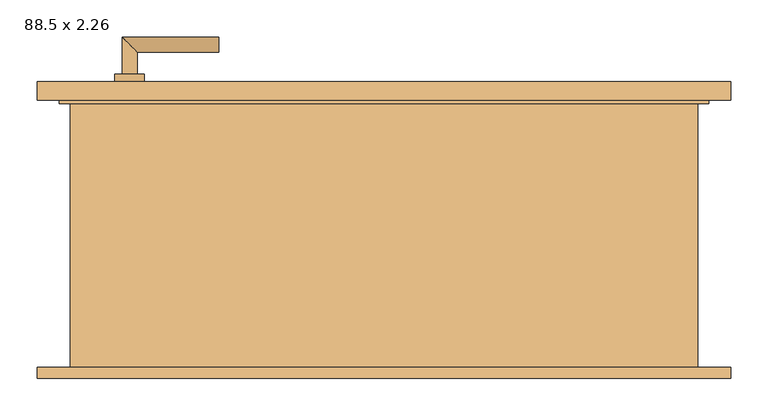
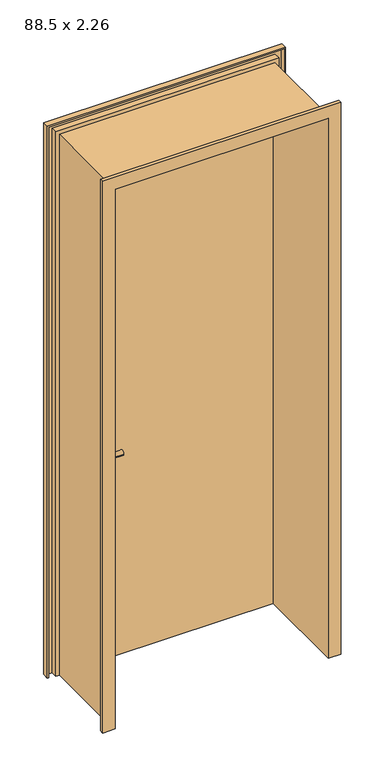
"""IFC4 building model written with IfcOpenShell, lengths in millimetres: door geometry, Drehflügel 1-flg - Stahlzarge : 88.5 x 2.26."""

from ifc_helpers import new_model, si_unit, point, frame, frame_2d, origin, place, context, project, spatial, polyline, circle_curve, ellipse_curve, trimmed, segment, composite_curve, outline, extrude, faceted_brep, source, transform, mapped, element, save
from ifc_brep_helpers import plane_surface, cylinder_surface, advanced_brep


def door_88_5_x_2_26_80f06d6c(model_context):
    return source(origin(), model_context, "Body", "SolidModel", [
        advanced_brep(
        [(-352.5, 169.4346141, 1000.0), (-332.5, 169.4346141, 1000.0), (-352.5, 99.4346141, 1000.0), (-332.5, 119.4346141, 1000.0), (-222.5, 99.4346141, 1000.0), (-222.5, 119.4346141, 1000.0)],
        [
            (0, 1, circle_curve(frame((-342.5, 169.4346141, 1000.0), z_axis=(0.0, 1.0, 0.0), x_axis=(1.0, 0.0, 0.0)), 10.0)),
            (1, 0, circle_curve(frame((-342.5, 169.4346141, 1000.0), z_axis=(0.0, 1.0, 0.0), x_axis=(1.0, 0.0, 0.0)), 10.0)),
            (0, 2),
            (2, 3, ellipse_curve(frame((-342.5, 109.4346141, 1000.0), z_axis=(-0.7071067811865385, 0.7071067811865565, 0.0), x_axis=(0.7071067811865563, 0.7071067811865386, 0.0)), 14.1421356, 10.0)),
            (3, 1),
            (3, 2, ellipse_curve(frame((-342.5, 109.4346141, 1000.0), z_axis=(-0.7071067811865385, 0.7071067811865565, 0.0), x_axis=(0.7071067811865563, 0.7071067811865386, 0.0)), 14.1421356, 10.0)),
            (4, 5, circle_curve(frame((-222.5, 109.4346141, 1000.0), z_axis=(1.0, 0.0, 0.0), x_axis=(0.0, 1.0, 0.0)), 10.0)),
            (5, 4, circle_curve(frame((-222.5, 109.4346141, 1000.0), z_axis=(1.0, 0.0, 0.0), x_axis=(0.0, 1.0, 0.0)), 10.0)),
            (2, 4),
            (5, 3),
        ],
        [
            plane_surface(frame((-342.5, 169.4346141, -287.7526403), z_axis=(0.0, 1.0, 0.0), x_axis=(0.0, 0.0, 1.0))),
            cylinder_surface(frame((-342.5, 169.4346141, 1000.0), z_axis=(0.0, 1.0, 0.0), x_axis=(1.0, 0.0, 0.0)), 10.0),
            plane_surface(frame((-222.5, 109.4346141, -287.7526403), z_axis=(1.0, 0.0, 0.0), x_axis=(0.0, 0.0, 1.0))),
            cylinder_surface(frame((-342.5, 109.4346141, 1000.0), z_axis=(-1.0, 0.0, 0.0), x_axis=(0.0, 1.0, 0.0)), 10.0),
        ],
        [
            (0, [[1, 2]]),
            (1, [[-1, 3, 4, 5]]),
            (1, [[-2, -5, 6, -3]]),
            (2, [[7, 8]]),
            (3, [[-4, 9, -8, 10]]),
            (3, [[-6, -10, -7, -9]]),
        ],
    ),
        advanced_brep(
        [(-332.5, 229.4346141, 1000.0), (-352.5, 229.4346141, 1000.0), (-332.5, 259.4346141, 1000.0), (-352.5, 279.4346141, 1000.0), (-222.5, 259.4346141, 1000.0), (-222.5, 279.4346141, 1000.0)],
        [
            (0, 1, circle_curve(frame((-342.5, 229.4346141, 1000.0), z_axis=(0.0, -1.0, 0.0), x_axis=(-1.0, 0.0, 0.0)), 10.0)),
            (1, 0, circle_curve(frame((-342.5, 229.4346141, 1000.0), z_axis=(0.0, -1.0, 0.0), x_axis=(-1.0, 0.0, 0.0)), 10.0)),
            (0, 2),
            (2, 3, ellipse_curve(frame((-342.5, 269.4346141, 1000.0), z_axis=(-0.7071067811865475, -0.7071067811865475, 0.0), x_axis=(0.7071067811865474, -0.7071067811865476, 0.0)), 14.1421356, 10.0)),
            (3, 1),
            (3, 2, ellipse_curve(frame((-342.5, 269.4346141, 1000.0), z_axis=(-0.7071067811865475, -0.7071067811865475, 0.0), x_axis=(0.7071067811865474, -0.7071067811865476, 0.0)), 14.1421356, 10.0)),
            (4, 5, circle_curve(frame((-222.5, 269.4346141, 1000.0), z_axis=(1.0, 0.0, 0.0), x_axis=(0.0, 1.0, 0.0)), 10.0)),
            (5, 4, circle_curve(frame((-222.5, 269.4346141, 1000.0), z_axis=(1.0, 0.0, 0.0), x_axis=(0.0, 1.0, 0.0)), 10.0)),
            (2, 4),
            (5, 3),
        ],
        [
            plane_surface(frame((-342.5, 229.4346141, -287.7526403), z_axis=(0.0, -1.0, 0.0), x_axis=(0.0, 0.0, 1.0))),
            cylinder_surface(frame((-342.5, 229.4346141, 1000.0), z_axis=(0.0, -1.0, 0.0), x_axis=(-1.0, 0.0, 0.0)), 10.0),
            plane_surface(frame((-222.5, 269.4346141, -287.7526403), z_axis=(1.0, 0.0, 0.0), x_axis=(0.0, 0.0, 1.0))),
            cylinder_surface(frame((-342.5, 269.4346141, 1000.0), z_axis=(-1.0, 0.0, 0.0), x_axis=(0.0, 1.0, 0.0)), 10.0),
        ],
        [
            (0, [[1, 2]]),
            (1, [[-1, 3, 4, 5]]),
            (1, [[-2, -5, 6, -3]]),
            (2, [[7, 8]]),
            (3, [[-4, 9, -8, 10]]),
            (3, [[-6, -10, -7, -9]]),
        ],
    ),
        extrude(outline(composite_curve([segment(trimmed(circle_curve(frame_2d((1000.0, -342.5)), 20.0), [point((1000.0, -362.5))], [point((1000.0, -322.5))], False, "CARTESIAN"), True, "CONTINUOUS"), segment(trimmed(circle_curve(frame_2d((1000.0, -342.5)), 20.0), [point((1000.0, -322.5))], [point((1000.0, -362.5))], False, "CARTESIAN"), True, "CONTINUOUS")], self_intersect=False)), frame((0.0, 159.4346141, 0.0), z_axis=(0.0, 1.0, 0.0), x_axis=(0.0, 0.0, 1.0)), (0.0, 0.0, 1.0), 10.0),
        extrude(outline(composite_curve([segment(trimmed(circle_curve(frame_2d((1000.0, -342.5)), 20.0), [point((1000.0, -362.5))], [point((1000.0, -322.5))], False, "CARTESIAN"), True, "CONTINUOUS"), segment(trimmed(circle_curve(frame_2d((1000.0, -342.5)), 20.0), [point((1000.0, -322.5))], [point((1000.0, -362.5))], False, "CARTESIAN"), True, "CONTINUOUS")], self_intersect=False)), frame((0.0, 219.4346141, 0.0), z_axis=(0.0, 1.0, 0.0), x_axis=(0.0, 0.0, 1.0)), (0.0, 0.0, 1.0), 10.0),
        extrude(outline(polyline([(432.5, 194.4346141), (-432.5, 194.4346141), (-432.5, 219.4346141), (432.5, 219.4346141), (432.5, 194.4346141)])), frame((0.0, 0.0, 100.0), z_axis=(0.0, 0.0, 1.0), x_axis=(1.0, 0.0, 0.0)), (0.0, 0.0, 1.0), 2250.0),
        faceted_brep([(466.9603207, -180.5653859, 100.0), (417.5, -180.5653859, 100.0), (417.5, 194.4346141, 100.0), (432.5, 194.4346141, 100.0), (432.5, 219.4346141, 100.0), (466.9603207, 219.4346141, 100.0), (466.9603207, 194.4346141, 100.0), (461.9603207, 194.4346141, 100.0), (461.9603207, 214.4346141, 100.0), (437.5, 214.4346141, 100.0), (437.5, 189.4346141, 100.0), (422.5, 189.4346141, 100.0), (422.5, -175.5653859, 100.0), (461.9603207, -175.5653859, 100.0), (461.9603207, -165.5653859, 100.0), (466.9603207, -165.5653859, 100.0), (466.9603207, -180.5653859, 2384.4603207), (-466.9603207, -180.5653859, 2384.4603207), (-466.9603207, -180.5653859, 100.0), (-417.5, -180.5653859, 100.0), (-417.5, -180.5653859, 2335.0), (417.5, -180.5653859, 2335.0), (417.5, 194.4346141, 2335.0), (-417.5, 194.4346141, 2335.0), (-417.5, 194.4346141, 100.0), (-432.5, 194.4346141, 100.0), (-432.5, 194.4346141, 2350.0), (432.5, 194.4346141, 2350.0), (432.5, 219.4346141, 2350.0), (-432.5, 219.4346141, 2350.0), (-432.5, 219.4346141, 100.0), (-466.9603207, 219.4346141, 100.0), (-466.9603207, 219.4346141, 2384.4603207), (466.9603207, 219.4346141, 2384.4603207), (466.9603207, 194.4346141, 2384.4603207), (-466.9603207, 194.4346141, 2384.4603207), (-466.9603207, 194.4346141, 100.0), (-461.9603207, 194.4346141, 100.0), (-461.9603207, 194.4346141, 2379.4603207), (461.9603207, 194.4346141, 2379.4603207), (461.9603207, 214.4346141, 2379.4603207), (-461.9603207, 214.4346141, 2379.4603207), (-461.9603207, 214.4346141, 100.0), (-437.5, 214.4346141, 100.0), (-437.5, 214.4346141, 2355.0), (437.5, 214.4346141, 2355.0), (437.5, 189.4346141, 2355.0), (-437.5, 189.4346141, 2355.0), (-437.5, 189.4346141, 100.0), (-422.5, 189.4346141, 100.0), (-422.5, 189.4346141, 2340.0), (422.5, 189.4346141, 2340.0), (422.5, -175.5653859, 2340.0), (-422.5, -175.5653859, 2340.0), (-422.5, -175.5653859, 100.0), (-461.9603207, -175.5653859, 100.0), (-461.9603207, -175.5653859, 2379.4603207), (461.9603207, -175.5653859, 2379.4603207), (461.9603207, -165.5653859, 2379.4603207), (-461.9603207, -165.5653859, 2379.4603207), (-461.9603207, -165.5653859, 100.0), (-466.9603207, -165.5653859, 100.0), (-466.9603207, -165.5653859, 2384.4603207), (466.9603207, -165.5653859, 2384.4603207)], [[[0, 1, 2, 3, 4, 5, 6, 7, 8, 9, 10, 11, 12, 13, 14, 15]], [[1, 0, 16, 17, 18, 19, 20, 21]], [[2, 1, 21, 22]], [[3, 2, 22, 23, 24, 25, 26, 27]], [[4, 3, 27, 28]], [[5, 4, 28, 29, 30, 31, 32, 33]], [[6, 5, 33, 34]], [[7, 6, 34, 35, 36, 37, 38, 39]], [[8, 7, 39, 40]], [[9, 8, 40, 41, 42, 43, 44, 45]], [[10, 9, 45, 46]], [[11, 10, 46, 47, 48, 49, 50, 51]], [[12, 11, 51, 52]], [[13, 12, 52, 53, 54, 55, 56, 57]], [[14, 13, 57, 58]], [[15, 14, 58, 59, 60, 61, 62, 63]], [[0, 15, 63, 16]], [[17, 62, 61, 18]], [[18, 61, 60, 55, 54, 49, 48, 43, 42, 37, 36, 31, 30, 25, 24, 19]], [[23, 20, 19, 24]], [[29, 26, 25, 30]], [[35, 32, 31, 36]], [[41, 38, 37, 42]], [[47, 44, 43, 48]], [[53, 50, 49, 54]], [[59, 56, 55, 60]], [[22, 21, 20, 23]], [[28, 27, 26, 29]], [[34, 33, 32, 35]], [[40, 39, 38, 41]], [[46, 45, 44, 47]], [[52, 51, 50, 53]], [[58, 57, 56, 59]], [[16, 63, 62, 17]]]),
    ])


if __name__ == "__main__":
    model = new_model("IFC4")
    model_context = context("Model", 3, world=origin())
    ifc_project = project(units=[si_unit("LENGTHUNIT", "METRE", prefix="MILLI")], contexts=[model_context])
    site = spatial("IfcSite", under=ifc_project)
    building = spatial("IfcBuilding", under=site)
    placement = place(None, origin())
    door_88_5_x_2_26_shape = door_88_5_x_2_26_80f06d6c(model_context)
    element("IfcDoor", 1, ObjectType="Drehflügel 1-flg - Stahlzarge : 88.5 x 2.26", at=placement, inside=building, context=model_context, shape_type="MappedRepresentation", body=[
        mapped(door_88_5_x_2_26_shape, transform((0.0, 0.0, 0.0), x_axis=(1.0, 0.0, 0.0), y_axis=(0.0, 1.0, 0.0), z_axis=(0.0, 0.0, 1.0))),
    ])
    save(model, "model.ifc")

# Revit data of these elements
# Type "Drehflügel 1-flg - Stahlzarge : 88.5 x 2.26"
#   Construction Type Id = "MDOOR"
#   Type Mark = "20"
#   Operation = "SingleSwingRight"
#   Keynote = "16.03"
#   Analytic Construction = "Metall"
#   Thermal Resistance (R) = 0.270117 (m²·K)/W
#   Heat Transfer Coefficient (U) = 3.7021 W/(m²·K)
#   Rough Width = 0.885 m
#   Rough Height [instance default] = 2.360 m
#   Höhe Türgriff [instance default] = 0.900 m
#   Height = 2.260 m
#   Fußbodenaufbau [instance default] = 0.100 m
#   Width = 0.885 m
#   Define Thermal Properties by = 1
#   Sichtbarkeit Sturzlinien [instance default] = yes
#   Türgriff auswählen [instance default] = element 221079
#   Türgriff [instance default] = none
#   Türflügel [instance default] = none
#   Rahmen/Pfosten [instance default] = Metall - Lackiert - Grau
#   Visual Light Transmittance = 0
#   Solar Heat Gain Coefficient = 0
#   Function = (empty or 0)
#   Wall Closure = (empty or 0)
# Element 1 (IfcDoor, "Drehflügel 1-flg - Stahlzarge : 88.5 x 2.26")
#   Materials on its faces: "Metall - Lackiert - Grau", "Metall - Chrom", "Holz - Birke"
# Materials
#   "Metall - Lackiert - Grau": class "Farbe 1", colour RGB 98 98 98, transparency 0, Cost = 0
#   "Metall - Chrom": class "Metall", colour RGB 247 247 247, transparency 0, Cost = 0
#   "Holz - Birke": class "Holz", colour RGB 213 164 103, transparency 0, Cost = 0
